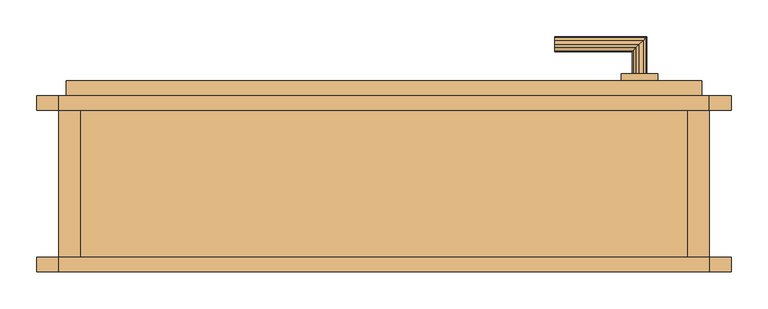
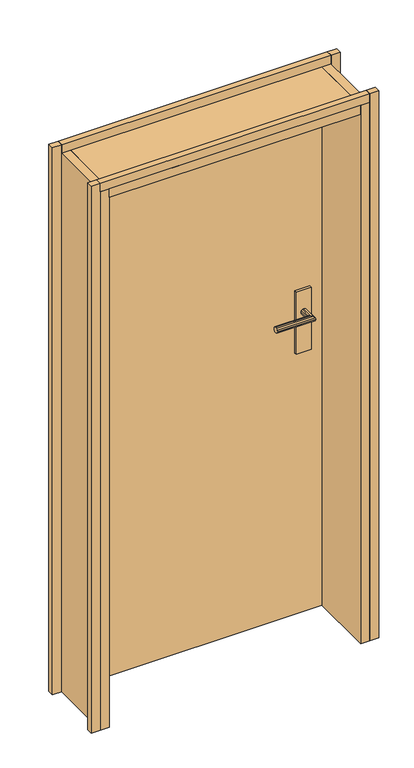
"""IFC4 building model written with IfcOpenShell, lengths in millimetres: door geometry, Tür."""

from ifc_helpers import new_model, si_unit, frame, origin, place, context, project, spatial, polyline, outline, extrude, faceted_brep, source, transform, mapped, element, save


def door_e7d93817(model_context):
    return source(origin(), model_context, "Body", "SolidModel", [
        extrude(outline(polyline([(855.0, 220.0), (855.0, -20.0), (30.0, -20.0), (30.0, 220.0), (855.0, 220.0)])), frame((0.0, 0.0, 1980.0), z_axis=(0.0, 0.0, 1.0), x_axis=(1.0, 0.0, 0.0)), (0.0, 0.0, 1.0), 30.0),
        extrude(outline(polyline([(815.0, 250.0), (815.0, 240.0), (765.0, 240.0), (765.0, 250.0), (815.0, 250.0)])), frame((0.0, 0.0, 1050.0), z_axis=(0.0, 0.0, 1.0), x_axis=(1.0, 0.0, 0.0)), (0.0, 0.0, 1.0), 215.0),
        faceted_brep([(795.0, 250.0, 1198.660254), (790.0, 250.0, 1200.0), (785.0, 250.0, 1198.660254), (781.339746, 250.0, 1195.0), (780.0, 250.0, 1190.0), (781.339746, 250.0, 1185.0), (785.0, 250.0, 1181.339746), (790.0, 250.0, 1180.0), (795.0, 250.0, 1181.339746), (798.660254, 250.0, 1185.0), (800.0, 250.0, 1190.0), (798.660254, 250.0, 1195.0), (790.0, 290.0, 1200.0), (795.0, 295.0, 1198.660254), (798.660254, 298.660254, 1195.0), (800.0, 300.0, 1190.0), (798.660254, 298.660254, 1185.0), (795.0, 295.0, 1181.339746), (790.0, 290.0, 1180.0), (785.0, 285.0, 1181.339746), (781.339746, 281.339746, 1185.0), (780.0, 280.0, 1190.0), (781.339746, 281.339746, 1195.0), (785.0, 285.0, 1198.660254), (675.0, 285.0, 1198.660254), (675.0, 290.0, 1200.0), (675.0, 295.0, 1198.660254), (675.0, 298.660254, 1195.0), (675.0, 300.0, 1190.0), (675.0, 298.660254, 1185.0), (675.0, 295.0, 1181.339746), (675.0, 290.0, 1180.0), (675.0, 285.0, 1181.339746), (675.0, 281.339746, 1185.0), (675.0, 280.0, 1190.0), (675.0, 281.339746, 1195.0)], [[[0, 1, 2, 3, 4, 5, 6, 7, 8, 9, 10, 11]], [[12, 1, 0, 13]], [[13, 0, 11, 14]], [[14, 11, 10, 15]], [[15, 10, 9, 16]], [[16, 9, 8, 17]], [[17, 8, 7, 18]], [[18, 7, 6, 19]], [[19, 6, 5, 20]], [[20, 5, 4, 21]], [[21, 4, 3, 22]], [[22, 3, 2, 23]], [[23, 2, 1, 12]], [[24, 25, 26, 27, 28, 29, 30, 31, 32, 33, 34, 35]], [[25, 12, 13, 26]], [[26, 13, 14, 27]], [[27, 14, 15, 28]], [[28, 15, 16, 29]], [[29, 16, 17, 30]], [[30, 17, 18, 31]], [[31, 18, 19, 32]], [[32, 19, 20, 33]], [[33, 20, 21, 34]], [[34, 21, 22, 35]], [[35, 22, 23, 24]], [[24, 23, 12, 25]]]),
        extrude(outline(polyline([(885.0, 0.0), (885.0, -20.0), (0.0, -20.0), (0.0, 0.0), (885.0, 0.0)])), frame((0.0, 0.0, 2010.0), z_axis=(0.0, 0.0, 1.0), x_axis=(1.0, 0.0, 0.0)), (0.0, 0.0, 1.0), 30.0),
        extrude(outline(polyline([(0.0, -20.0), (-30.0, -20.0), (-30.0, 0.0), (0.0, 0.0), (0.0, -20.0)])), frame((0.0, 0.0, 140.0), z_axis=(0.0, 0.0, 1.0), x_axis=(1.0, 0.0, 0.0)), (0.0, 0.0, 1.0), 1900.0),
        extrude(outline(polyline([(30.0, 220.0), (30.0, -20.0), (0.0, -20.0), (0.0, 220.0), (30.0, 220.0)])), frame((0.0, 0.0, 140.0), z_axis=(0.0, 0.0, 1.0), x_axis=(1.0, 0.0, 0.0)), (0.0, 0.0, 1.0), 1870.0),
        extrude(outline(polyline([(885.0, 220.0), (885.0, -20.0), (855.0, -20.0), (855.0, 220.0), (885.0, 220.0)])), frame((0.0, 0.0, 140.0), z_axis=(0.0, 0.0, 1.0), x_axis=(1.0, 0.0, 0.0)), (0.0, 0.0, 1.0), 1870.0),
        extrude(outline(polyline([(915.0, 220.0), (915.0, 200.0), (885.0, 200.0), (885.0, 220.0), (915.0, 220.0)])), frame((0.0, 0.0, 140.0), z_axis=(0.0, 0.0, 1.0), x_axis=(1.0, 0.0, 0.0)), (0.0, 0.0, 1.0), 1900.0),
        faceted_brep([(785.0, 190.0, 1198.660254), (790.0, 190.0, 1200.0), (795.0, 190.0, 1198.660254), (798.660254, 190.0, 1195.0), (800.0, 190.0, 1190.0), (798.660254, 190.0, 1185.0), (795.0, 190.0, 1181.339746), (790.0, 190.0, 1180.0), (785.0, 190.0, 1181.339746), (781.339746, 190.0, 1185.0), (780.0, 190.0, 1190.0), (781.339746, 190.0, 1195.0), (790.0, 150.0, 1200.0), (795.0, 145.0, 1198.660254), (798.660254, 141.339746, 1195.0), (800.0, 140.0, 1190.0), (798.660254, 141.339746, 1185.0), (795.0, 145.0, 1181.339746), (790.0, 150.0, 1180.0), (785.0, 155.0, 1181.339746), (781.339746, 158.660254, 1185.0), (780.0, 160.0, 1190.0), (781.339746, 158.660254, 1195.0), (785.0, 155.0, 1198.660254), (675.0, 145.0, 1198.660254), (675.0, 150.0, 1200.0), (675.0, 155.0, 1198.660254), (675.0, 158.660254, 1195.0), (675.0, 160.0, 1190.0), (675.0, 158.660254, 1185.0), (675.0, 155.0, 1181.339746), (675.0, 150.0, 1180.0), (675.0, 145.0, 1181.339746), (675.0, 141.339746, 1185.0), (675.0, 140.0, 1190.0), (675.0, 141.339746, 1195.0)], [[[0, 1, 2, 3, 4, 5, 6, 7, 8, 9, 10, 11]], [[2, 1, 12, 13]], [[3, 2, 13, 14]], [[4, 3, 14, 15]], [[5, 4, 15, 16]], [[6, 5, 16, 17]], [[7, 6, 17, 18]], [[8, 7, 18, 19]], [[9, 8, 19, 20]], [[10, 9, 20, 21]], [[11, 10, 21, 22]], [[0, 11, 22, 23]], [[1, 0, 23, 12]], [[24, 25, 26, 27, 28, 29, 30, 31, 32, 33, 34, 35]], [[13, 12, 25, 24]], [[14, 13, 24, 35]], [[15, 14, 35, 34]], [[16, 15, 34, 33]], [[17, 16, 33, 32]], [[18, 17, 32, 31]], [[19, 18, 31, 30]], [[20, 19, 30, 29]], [[21, 20, 29, 28]], [[22, 21, 28, 27]], [[23, 22, 27, 26]], [[12, 23, 26, 25]]]),
        extrude(outline(polyline([(875.0, 240.0), (875.0, 200.0), (10.0, 200.0), (10.0, 240.0), (875.0, 240.0)])), frame((0.0, 0.0, 140.0), z_axis=(0.0, 0.0, 1.0), x_axis=(1.0, 0.0, 0.0)), (0.0, 0.0, 1.0), 1860.0),
        extrude(outline(polyline([(885.0, 220.0), (885.0, 200.0), (0.0, 200.0), (0.0, 220.0), (885.0, 220.0)])), frame((0.0, 0.0, 2010.0), z_axis=(0.0, 0.0, 1.0), x_axis=(1.0, 0.0, 0.0)), (0.0, 0.0, 1.0), 30.0),
        extrude(outline(polyline([(765.0, 200.0), (815.0, 200.0), (815.0, 190.0), (765.0, 190.0), (765.0, 200.0)])), frame((0.0, 0.0, 1050.0), z_axis=(0.0, 0.0, 1.0), x_axis=(1.0, 0.0, 0.0)), (0.0, 0.0, 1.0), 215.0),
        extrude(outline(polyline([(0.0, 200.0), (-30.0, 200.0), (-30.0, 220.0), (0.0, 220.0), (0.0, 200.0)])), frame((0.0, 0.0, 140.0), z_axis=(0.0, 0.0, 1.0), x_axis=(1.0, 0.0, 0.0)), (0.0, 0.0, 1.0), 1900.0),
        extrude(outline(polyline([(915.0, 0.0), (915.0, -20.0), (885.0, -20.0), (885.0, 0.0), (915.0, 0.0)])), frame((0.0, 0.0, 140.0), z_axis=(0.0, 0.0, 1.0), x_axis=(1.0, 0.0, 0.0)), (0.0, 0.0, 1.0), 1900.0),
    ])


if __name__ == "__main__":
    model = new_model("IFC4")
    model_context = context("Model", 3, world=origin())
    ifc_project = project(units=[si_unit("LENGTHUNIT", "METRE", prefix="MILLI")], contexts=[model_context])
    site = spatial("IfcSite", under=ifc_project)
    building = spatial("IfcBuilding", under=site)
    placement = place(None, origin())
    door_shape = door_e7d93817(model_context)
    element("IfcDoor", 1, ObjectType="Tür", at=placement, inside=building, context=model_context, shape_type="MappedRepresentation", body=[
        mapped(door_shape, transform((0.0, 0.0, 0.0), x_axis=(1.0, 0.0, 0.0), y_axis=(0.0, 1.0, 0.0), z_axis=(0.0, 0.0, 1.0))),
    ])
    save(model, "model.ifc")

# Revit data of these elements
# Type "Tür"
#   Type Mark = "44"
# Element 1 (IfcDoor, "Tür")
#   Materials on its faces: "tuer_beschlag", "tuer_holzzarge"
# Materials
#   "tuer_beschlag": class "Unassigned", colour RGB 128 128 128, transparency 0
#   "tuer_holzzarge": class "Unassigned", colour RGB 255 255 255, transparency 0
